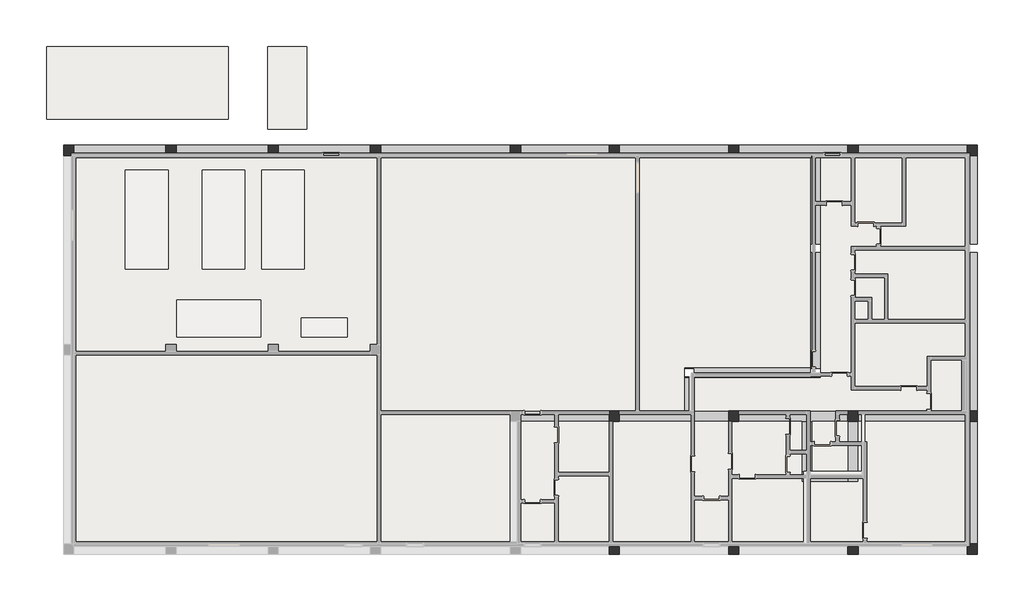
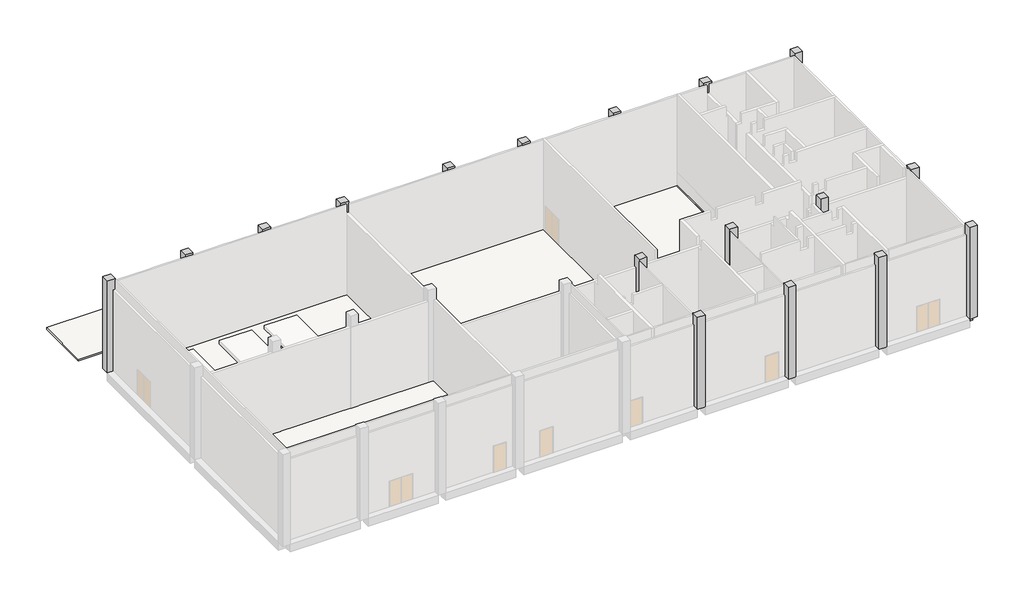
# One storey, part 4 of 4: 17 columns, 9 beams, 3 slabs.
"""IFC4 building model written with IfcOpenShell, lengths in millimetres."""

from ifc_helpers import new_model, si_unit, frame, origin, place, context, project, spatial, polyline, outline, extrude, faceted_brep, element, save

model = new_model("IFC4")

# Units and contexts
model_context = context("Model", 3, world=origin())
ifc_project = project(units=[si_unit("LENGTHUNIT", "METRE", prefix="MILLI")], contexts=[model_context])

# Site, building, storey
site = spatial("IfcSite", under=ifc_project)
building = spatial("IfcBuilding", under=site)
storey = spatial("IfcBuildingStorey", under=building, Name="TOC(GF)", Elevation=97049.9618634)

# Beams
placement = place(None, origin())
element("IfcBeam", 1, ObjectType="RC Beam_Rectangular : H_SB_AR S16_TG-UG_TG1 600x650", at=placement, inside=storey, context=model_context, shape_type="Brep", body=[
    faceted_brep([(5700.0, 3600.0, 97049.9618634), (5700.0, 4200.0, 97049.9618634), (300.0, 4200.0, 97049.9618634), (300.0, 3600.0, 97049.9618634), (5700.0, 4200.0, 96399.9618634), (300.0, 4200.0, 96399.9618634), (5700.0, 3600.0, 96399.9618634), (300.0, 3600.0, 96399.9618634), (300.0, 3600.0, 96849.9618634)], [[[0, 1, 2, 3]], [[1, 4, 5, 2]], [[4, 6, 7, 5]], [[6, 0, 3, 8, 7]], [[3, 2, 5, 7, 8]], [[1, 0, 6, 4]]]),
    faceted_brep([(6300.0, 3600.0, 97049.9618634), (6300.0, 4200.0, 97049.9618634), (6300.0, 4200.0, 96399.9618634), (6300.0, 3600.0, 96399.9618634), (11700.0, 4200.0, 97049.9618634), (11700.0, 3600.0, 97049.9618634), (11700.0, 3600.0, 96399.9618634), (11700.0, 4200.0, 96399.9618634)], [[[0, 1, 2, 3]], [[4, 5, 6, 7]], [[1, 0, 5, 4]], [[2, 1, 4, 7]], [[3, 2, 7, 6]], [[0, 3, 6, 5]]]),
    faceted_brep([(12300.0, 3600.0, 97049.9618634), (12300.0, 4200.0, 97049.9618634), (12300.0, 4200.0, 96399.9618634), (12300.0, 3600.0, 96399.9618634), (17700.0, 4200.0, 97049.9618634), (17700.0, 3600.0, 97049.9618634), (17700.0, 3600.0, 96399.9618634), (17700.0, 4200.0, 96399.9618634)], [[[0, 1, 2, 3]], [[4, 5, 6, 7]], [[1, 0, 5, 4]], [[2, 1, 4, 7]], [[3, 2, 7, 6]], [[0, 3, 6, 5]]]),
    faceted_brep([(18300.0, 3600.0, 97049.9618634), (18300.0, 4200.0, 97049.9618634), (18300.0, 4200.0, 96399.9618634), (18300.0, 3600.0, 96399.9618634), (25900.0, 3600.0, 97049.9618634), (25900.0, 4200.0, 97049.9618634), (25900.0, 4200.0, 96399.9618634), (25900.0, 3600.0, 96399.9618634)], [[[0, 1, 2, 3]], [[1, 0, 4, 5]], [[2, 1, 5, 6]], [[3, 2, 6, 7]], [[0, 3, 7, 4]], [[5, 4, 7, 6]]]),
    faceted_brep([(52700.0, 4200.0, 97049.9618634), (52700.0, 3600.0, 97049.9618634), (52700.0, 3600.0, 96849.9618634), (52700.0, 3600.0, 96399.9618634), (52700.0, 4200.0, 96399.9618634), (46300.0, 3600.0, 97049.9618634), (46300.0, 4200.0, 97049.9618634), (46300.0, 4200.0, 96399.9618634), (46300.0, 3600.0, 96399.9618634)], [[[0, 1, 2, 3, 4]], [[5, 6, 7, 8]], [[1, 0, 6, 5]], [[0, 4, 7, 6]], [[4, 3, 8, 7]], [[3, 2, 1, 5, 8]]]),
    faceted_brep([(45700.0, 4200.0, 97049.9618634), (45700.0, 3600.0, 97049.9618634), (45700.0, 3600.0, 96399.9618634), (45700.0, 4200.0, 96399.9618634), (39300.0, 3600.0, 97049.9618634), (39300.0, 4200.0, 97049.9618634), (39300.0, 4200.0, 96399.9618634), (39300.0, 3600.0, 96399.9618634), (43500.0, 3600.0, 97049.9618634), (44100.0, 3600.0, 97049.9618634), (44100.0, 3600.0, 96399.9618634), (43500.0, 3600.0, 96399.9618634)], [[[0, 1, 2, 3]], [[4, 5, 6, 7]], [[1, 0, 5, 4, 8, 9]], [[0, 3, 6, 5]], [[3, 2, 10, 11, 7, 6]], [[2, 1, 9, 8, 4, 7, 11, 10]]]),
    faceted_brep([(38700.0, 4200.0, 97049.9618634), (38700.0, 3600.0, 97049.9618634), (38700.0, 3600.0, 96399.9618634), (38700.0, 4200.0, 96399.9618634), (32300.0, 3600.0, 97049.9618634), (32300.0, 4200.0, 97049.9618634), (32300.0, 4200.0, 96399.9618634), (32300.0, 3600.0, 96399.9618634)], [[[0, 1, 2, 3]], [[4, 5, 6, 7]], [[1, 0, 5, 4]], [[0, 3, 6, 5]], [[3, 2, 7, 6]], [[2, 1, 4, 7]]]),
    faceted_brep([(31700.0, 4200.0, 97049.9618634), (31700.0, 3600.0, 97049.9618634), (31700.0, 3600.0, 96399.9618634), (31700.0, 4200.0, 96399.9618634), (26500.0, 3600.0, 97049.9618634), (26500.0, 4200.0, 97049.9618634), (26500.0, 4200.0, 96399.9618634), (26500.0, 3600.0, 96399.9618634)], [[[0, 1, 2, 3]], [[4, 5, 6, 7]], [[1, 0, 5, 4]], [[0, 3, 6, 5]], [[3, 2, 7, 6]], [[2, 1, 4, 7]]]),
])
element("IfcBeam", 2, ObjectType="RC Beam_Rectangular : H_SB_AR S16_TG-UG_TG1 600x650", at=placement, inside=storey, context=model_context, shape_type="Brep", body=[
    faceted_brep([(53300.0, 3600.0, 97049.9618634), (52700.0, 3600.0, 97049.9618634), (52700.0, -1600.0, 97049.9618634), (53300.0, -1600.0, 97049.9618634), (53300.0, -1600.0, 96399.9618634), (53300.0, 3600.0, 96399.9618634), (52700.0, 3600.0, 96399.9618634), (52700.0, -1600.0, 96399.9618634), (52700.0, 3600.0, 96849.9618634)], [[[0, 1, 2, 3]], [[3, 4, 5, 0]], [[6, 5, 4, 7]], [[1, 8, 6, 7, 2]], [[0, 5, 6, 8, 1]], [[3, 2, 7, 4]]]),
    faceted_brep([(52700.0, -19200.0, 97049.9618634), (52700.0, -19200.0, 96849.9618634), (52700.0, -19200.0, 96399.9618634), (53300.0, -19200.0, 96399.9618634), (53300.0, -19200.0, 97049.9618634), (52700.0, -12000.0, 97049.9618634), (53300.0, -12000.0, 97049.9618634), (53300.0, -12000.0, 96399.9618634), (52700.0, -12000.0, 96399.9618634), (52700.0, -12000.0, 96849.9618634)], [[[0, 1, 2, 3, 4]], [[5, 6, 7, 8, 9]], [[0, 4, 6, 5]], [[4, 3, 7, 6]], [[3, 2, 8, 7]], [[2, 1, 0, 5, 9, 8]]]),
    faceted_brep([(52700.0, -2100.0, 97049.9618634), (53300.0, -2100.0, 97049.9618634), (53300.0, -2100.0, 96399.9618634), (52700.0, -2100.0, 96399.9618634), (52700.0, -11400.0, 97049.9618634), (53300.0, -11400.0, 97049.9618634), (53300.0, -11400.0, 96399.9618634), (52700.0, -11400.0, 96399.9618634), (52700.0, -11400.0, 96849.9618634)], [[[0, 1, 2, 3]], [[1, 0, 4, 5]], [[2, 1, 5, 6]], [[3, 2, 6, 7]], [[0, 3, 7, 8, 4]], [[5, 4, 8, 7, 6]]]),
])
element("IfcBeam", 3, ObjectType="RC Beam_Rectangular : H_SB_AR S16_TG-UG_TG1 600x650", at=placement, inside=storey, context=model_context, shape_type="Brep", body=[
    faceted_brep([(43500.0, -9450.0, 97049.9618634), (44100.0, -9450.0, 97049.9618634), (44100.0, -9400.0, 97049.9618634), (43500.0, -9400.0, 97049.9618634), (43500.0, -9450.0, 96399.9618634), (43500.0, -9400.0, 96399.9618634), (44100.0, -9450.0, 96399.9618634), (44100.0, -9400.0, 96399.9618634), (44100.0, -9450.0, 96849.9618634)], [[[0, 1, 2, 3]], [[4, 0, 3, 5]], [[6, 4, 5, 7]], [[1, 8, 6, 7, 2]], [[1, 0, 4, 6, 8]], [[3, 2, 7, 5]]]),
    faceted_brep([(43500.0, 3600.0, 97049.9618634), (44100.0, 3600.0, 97049.9618634), (44100.0, 3600.0, 96849.9618634), (44100.0, 3600.0, 96399.9618634), (43500.0, 3600.0, 96399.9618634), (43500.0, 3600.0, 96849.9618634), (44100.0, -1600.0, 97049.9618634), (43500.0, -1600.0, 97049.9618634), (43500.0, -1600.0, 96399.9618634), (44100.0, -1600.0, 96399.9618634)], [[[0, 1, 2, 3, 4, 5]], [[6, 7, 8, 9]], [[1, 0, 7, 6]], [[0, 5, 4, 8, 7]], [[4, 3, 9, 8]], [[3, 2, 1, 6, 9]]]),
    faceted_brep([(43500.0, -2100.0, 97049.9618634), (44100.0, -2100.0, 97049.9618634), (44100.0, -2100.0, 96399.9618634), (43500.0, -2100.0, 96399.9618634), (44100.0, -8900.0, 97049.9618634), (43500.0, -8900.0, 97049.9618634), (43500.0, -8900.0, 96399.9618634), (44100.0, -8900.0, 96399.9618634), (43500.0, -8850.0, 97049.9618634), (43500.0, -8850.0, 96399.9618634)], [[[0, 1, 2, 3]], [[4, 5, 6, 7]], [[1, 0, 8, 5, 4]], [[0, 3, 9, 6, 5, 8]], [[3, 2, 7, 6, 9]], [[2, 1, 4, 7]]]),
])
element("IfcBeam", 4, ObjectType="RC Beam_Rectangular : H_SB_AR S16_TG-UG_TG1 600x650", at=placement, inside=storey, context=model_context, shape_type="Brep", body=[
    faceted_brep([(43500.0, -9450.0, 97049.9618634), (43500.0, -9400.0, 97049.9618634), (43500.0, -8900.0, 97049.9618634), (43500.0, -8850.0, 97049.9618634), (36100.0, -8850.0, 97049.9618634), (36100.0, -8900.0, 97049.9618634), (36700.0, -8900.0, 97049.9618634), (36700.0, -9400.0, 97049.9618634), (36100.0, -9400.0, 97049.9618634), (36100.0, -9450.0, 97049.9618634), (36700.0, -9450.0, 97049.9618634), (43500.0, -8850.0, 96849.9618634), (43500.0, -8850.0, 96399.9618634), (36100.0, -8850.0, 96399.9618634), (36100.0, -8850.0, 96849.9618634), (43500.0, -8900.0, 96399.9618634), (43500.0, -9400.0, 96399.9618634), (43500.0, -9450.0, 96399.9618634), (36700.0, -9450.0, 96399.9618634), (36100.0, -9450.0, 96399.9618634), (36100.0, -9400.0, 96399.9618634), (36700.0, -9400.0, 96399.9618634), (36700.0, -8900.0, 96399.9618634), (36100.0, -8900.0, 96399.9618634)], [[[0, 1, 2, 3, 4, 5, 6, 7, 8, 9, 10]], [[3, 11, 12, 13, 14, 4]], [[12, 15, 16, 17, 18, 19, 20, 21, 22, 23, 13]], [[9, 19, 18, 17, 0, 10]], [[3, 2, 1, 0, 17, 16, 15, 12, 11]], [[7, 21, 20, 8]], [[22, 6, 5, 23]], [[6, 22, 21, 7]], [[4, 14, 13, 23, 5]], [[19, 9, 8, 20]]]),
])
element("IfcBeam", 5, ObjectType="RC Beam_Rectangular : H_SB_AR S16_TG-UG_TG1 600x650", at=placement, inside=storey, context=model_context, shape_type="Brep", body=[
    faceted_brep([(26500.0, -11400.0, 97049.9618634), (26500.0, -12000.0, 97049.9618634), (31700.0, -12000.0, 97049.9618634), (31700.0, -11400.0, 97049.9618634), (26500.0, -12000.0, 96849.9618634), (26500.0, -12000.0, 96399.9618634), (31700.0, -12000.0, 96399.9618634), (26500.0, -11400.0, 96399.9618634), (31700.0, -11400.0, 96399.9618634)], [[[0, 1, 2, 3]], [[1, 4, 5, 6, 2]], [[5, 7, 8, 6]], [[7, 0, 3, 8]], [[1, 0, 7, 5, 4]], [[3, 2, 6, 8]]]),
    faceted_brep([(32300.0, -12000.0, 97049.9618634), (32300.0, -11400.0, 97049.9618634), (32300.0, -11400.0, 96399.9618634), (32300.0, -12000.0, 96399.9618634), (38700.0, -11400.0, 97049.9618634), (38700.0, -12000.0, 97049.9618634), (38700.0, -12000.0, 96399.9618634), (38700.0, -11400.0, 96399.9618634), (36700.0, -11400.0, 97049.9618634), (36100.0, -11400.0, 97049.9618634), (36100.0, -11400.0, 96399.9618634), (36700.0, -11400.0, 96399.9618634)], [[[0, 1, 2, 3]], [[4, 5, 6, 7]], [[1, 0, 5, 4, 8, 9]], [[0, 3, 6, 5]], [[3, 2, 10, 11, 7, 6]], [[2, 1, 9, 8, 4, 7, 11, 10]]]),
    faceted_brep([(39300.0, -12000.0, 97049.9618634), (39300.0, -11400.0, 97049.9618634), (39300.0, -11400.0, 96399.9618634), (39300.0, -12000.0, 96399.9618634), (45700.0, -11400.0, 97049.9618634), (45700.0, -12000.0, 97049.9618634), (45700.0, -12000.0, 96849.9618634), (45700.0, -12000.0, 96399.9618634), (45700.0, -11400.0, 96399.9618634), (43000.0, -12000.0, 97049.9618634), (43600.0, -12000.0, 97049.9618634), (43000.0, -12000.0, 96399.9618634), (43600.0, -12000.0, 96399.9618634)], [[[0, 1, 2, 3]], [[4, 5, 6, 7, 8]], [[4, 1, 0, 9, 10, 5]], [[5, 10, 9, 0, 3, 11, 12, 7, 6]], [[7, 12, 11, 3, 2, 8]], [[1, 4, 8, 2]]]),
    faceted_brep([(46300.0, -12000.0, 97049.9618634), (46300.0, -11400.0, 97049.9618634), (46300.0, -11400.0, 96399.9618634), (46300.0, -12000.0, 96399.9618634), (46300.0, -12000.0, 96849.9618634), (52700.0, -11400.0, 97049.9618634), (52700.0, -12000.0, 97049.9618634), (52700.0, -12000.0, 96849.9618634), (52700.0, -12000.0, 96399.9618634), (52700.0, -11400.0, 96399.9618634), (52700.0, -11400.0, 96849.9618634)], [[[0, 1, 2, 3, 4]], [[5, 6, 7, 8, 9, 10]], [[1, 0, 6, 5]], [[0, 4, 3, 8, 7, 6]], [[3, 2, 9, 8]], [[2, 1, 5, 10, 9]]]),
])
element("IfcBeam", 6, ObjectType="RC Beam_Rectangular : H_SB_AR S16_TG-UG_TG1 600x650", at=placement, inside=storey, context=model_context, shape_type="Brep", body=[
    faceted_brep([(36700.0, -9450.0, 97049.9618634), (36100.0, -9450.0, 97049.9618634), (36100.0, -11400.0, 97049.9618634), (36700.0, -11400.0, 97049.9618634), (36100.0, -9450.0, 96399.9618634), (36100.0, -11400.0, 96399.9618634), (36100.0, -11400.0, 96849.9618634), (36700.0, -9450.0, 96399.9618634), (36700.0, -11400.0, 96399.9618634), (36700.0, -9450.0, 96849.9618634), (36700.0, -11400.0, 96849.9618634)], [[[0, 1, 2, 3]], [[1, 4, 5, 6, 2]], [[4, 7, 8, 5]], [[7, 9, 0, 3, 10, 8]], [[1, 0, 9, 7, 4]], [[3, 2, 6, 5, 8, 10]]]),
])
element("IfcBeam", 7, ObjectType="RC Beam_Rectangular : H_SB_AR S16_TG-UG_TG1 600x650", at=placement, inside=storey, context=model_context, shape_type="Brep", body=[
    faceted_brep([(45700.0, -15550.0, 97049.9618634), (46300.0, -15550.0, 97049.9618634), (46300.0, -12000.0, 97049.9618634), (45700.0, -12000.0, 97049.9618634), (45700.0, -14950.0, 97049.9618634), (45700.0, -15550.0, 96399.9618634), (45700.0, -12000.0, 96849.9618634), (45700.0, -12000.0, 96399.9618634), (45700.0, -14950.0, 96399.9618634), (46300.0, -15550.0, 96399.9618634), (46300.0, -12000.0, 96399.9618634), (46300.0, -15550.0, 96849.9618634), (46300.0, -12000.0, 96849.9618634)], [[[0, 1, 2, 3, 4]], [[5, 0, 4, 3, 6, 7, 8]], [[9, 5, 8, 7, 10]], [[1, 11, 9, 10, 12, 2]], [[1, 0, 5, 9, 11]], [[3, 2, 12, 10, 7, 6]]]),
])
element("IfcBeam", 8, ObjectType="RC Beam_Rectangular : H_SB_AR S16_TG-UG_TG1 600x650", at=placement, inside=storey, context=model_context, shape_type="Brep", body=[
    faceted_brep([(43000.0, -14950.0, 97049.9618634), (43000.0, -15550.0, 97049.9618634), (45700.0, -15550.0, 97049.9618634), (45700.0, -14950.0, 97049.9618634), (43600.0, -14950.0, 97049.9618634), (43000.0, -14950.0, 96399.9618634), (45700.0, -14950.0, 96849.9618634), (45700.0, -14950.0, 96399.9618634), (43600.0, -14950.0, 96399.9618634), (43000.0, -15550.0, 96399.9618634), (45700.0, -15550.0, 96399.9618634), (43000.0, -15550.0, 96849.9618634)], [[[0, 1, 2, 3, 4]], [[5, 0, 4, 3, 6, 7, 8]], [[9, 5, 8, 7, 10]], [[1, 11, 9, 10, 2]], [[3, 2, 10, 7, 6]], [[1, 0, 5, 9, 11]]]),
])
element("IfcBeam", 9, ObjectType="RC Beam_Rectangular : H_SB_AR S16_TG-UG_TG1 600x650", at=placement, inside=storey, context=model_context, shape_type="Brep", body=[
    faceted_brep([(43000.0, -14950.0, 97049.9618634), (43600.0, -14950.0, 97049.9618634), (43600.0, -12000.0, 97049.9618634), (43000.0, -12000.0, 97049.9618634), (43600.0, -14950.0, 96849.9618634), (43600.0, -14950.0, 96399.9618634), (43600.0, -12000.0, 96399.9618634), (43600.0, -12000.0, 96849.9618634), (43000.0, -14950.0, 96399.9618634), (43000.0, -12000.0, 96399.9618634), (43000.0, -12000.0, 96849.9618634)], [[[0, 1, 2, 3]], [[1, 4, 5, 6, 7, 2]], [[5, 8, 9, 6]], [[8, 0, 3, 10, 9]], [[1, 0, 8, 5, 4]], [[3, 2, 7, 6, 9, 10]]]),
])

# Columns
element("IfcColumn", 10, ObjectType="RC_Column_Rectangular : H_SC_AR S15_RC Col-AG_C1 600x600", at=placement, inside=storey, context=model_context, shape_type="Brep", body=[
    faceted_brep([(300.0, 4200.0, 97049.9618634), (300.0, 3600.0, 97049.9618634), (-300.0, 3600.0, 97049.9618634), (-300.0, 4200.0, 97049.9618634), (300.0, 4200.0, 104550.0), (300.0, 3600.0, 104550.0), (300.0, 3600.0, 103650.0), (300.0, 4200.0, 103650.0), (-300.0, 3600.0, 104550.0), (-300.0, 3600.0, 103650.0), (-300.0, 4200.0, 104550.0)], [[[0, 1, 2, 3]], [[4, 5, 6, 1, 0, 7]], [[5, 8, 9, 2, 1, 6]], [[8, 10, 3, 2, 9]], [[10, 4, 7, 0, 3]], [[4, 10, 8, 5]]]),
])
element("IfcColumn", 11, ObjectType="RC_Column_Rectangular : H_SC_AR S15_RC Col-AG_C1 600x600", at=placement, inside=storey, context=model_context, shape_type="Brep", body=[
    faceted_brep([(32300.0, -19200.0, 97049.9618634), (32300.0, -19800.0, 97049.9618634), (31700.0, -19800.0, 97049.9618634), (31700.0, -19200.0, 97049.9618634), (32300.0, -19200.0, 104550.0), (32300.0, -19800.0, 104550.0), (32300.0, -19800.0, 103650.0), (32300.0, -19200.0, 103650.0), (31700.0, -19800.0, 104550.0), (31700.0, -19800.0, 103650.0), (31700.0, -19200.0, 104550.0), (31700.0, -19200.0, 103650.0), (31750.0, -19200.0, 104550.0), (32250.0, -19200.0, 104550.0)], [[[0, 1, 2, 3]], [[4, 5, 6, 1, 0, 7]], [[5, 8, 9, 2, 1, 6]], [[8, 10, 11, 3, 2, 9]], [[10, 12, 13, 4, 7, 0, 3, 11]], [[4, 13, 12, 10, 8, 5]]]),
])
element("IfcColumn", 12, ObjectType="RC_Column_Rectangular : H_SC_AR S15_RC Col-AG_C1 600x600", at=placement, inside=storey, context=model_context, shape_type="Brep", body=[
    faceted_brep([(39300.0, -19200.0, 97049.9618634), (39300.0, -19800.0, 97049.9618634), (38700.0, -19800.0, 97049.9618634), (38700.0, -19200.0, 97049.9618634), (39300.0, -19200.0, 104550.0), (39300.0, -19800.0, 104550.0), (39300.0, -19800.0, 103650.0), (39300.0, -19200.0, 103650.0), (38700.0, -19800.0, 104550.0), (38700.0, -19800.0, 103650.0), (38700.0, -19200.0, 104550.0), (38700.0, -19200.0, 103650.0), (38750.0, -19200.0, 104550.0), (39250.0, -19200.0, 104550.0)], [[[0, 1, 2, 3]], [[4, 5, 6, 1, 0, 7]], [[5, 8, 9, 2, 1, 6]], [[8, 10, 11, 3, 2, 9]], [[10, 12, 13, 4, 7, 0, 3, 11]], [[4, 13, 12, 10, 8, 5]]]),
])
element("IfcColumn", 13, ObjectType="RC_Column_Rectangular : H_SC_AR S15_RC Col-AG_C1 600x600", at=placement, inside=storey, context=model_context, shape_type="Brep", body=[
    faceted_brep([(46300.0, -19200.0, 97049.9618634), (46300.0, -19800.0, 97049.9618634), (45700.0, -19800.0, 97049.9618634), (45700.0, -19200.0, 97049.9618634), (46300.0, -19200.0, 104550.0), (46300.0, -19800.0, 104550.0), (46300.0, -19800.0, 103650.0), (46300.0, -19200.0, 103650.0), (45700.0, -19800.0, 104550.0), (45700.0, -19800.0, 103650.0), (45700.0, -19200.0, 104550.0), (45700.0, -19200.0, 103650.0), (45750.0, -19200.0, 104550.0), (46250.0, -19200.0, 104550.0)], [[[0, 1, 2, 3]], [[4, 5, 6, 1, 0, 7]], [[5, 8, 9, 2, 1, 6]], [[8, 10, 11, 3, 2, 9]], [[10, 12, 13, 4, 7, 0, 3, 11]], [[4, 13, 12, 10, 8, 5]]]),
])
element("IfcColumn", 14, ObjectType="RC_Column_Rectangular : H_SC_AR S15_RC Col-AG_C1 600x600", at=placement, inside=storey, context=model_context, shape_type="Brep", body=[
    faceted_brep([(53300.0, -19200.0, 97049.9618634), (53300.0, -19800.0, 97049.9618634), (52700.0, -19800.0, 97049.9618634), (52700.0, -19200.0, 97049.9618634), (53300.0, -19200.0, 104550.0), (53300.0, -19800.0, 104550.0), (53300.0, -19200.0, 103650.0), (52700.0, -19800.0, 104550.0), (52700.0, -19800.0, 103650.0), (52700.0, -19200.0, 104550.0), (52700.0, -19200.0, 103650.0)], [[[0, 1, 2, 3]], [[4, 5, 1, 0, 6]], [[5, 7, 8, 2, 1]], [[7, 9, 10, 3, 2, 8]], [[9, 4, 6, 0, 3, 10]], [[4, 9, 7, 5]]]),
])
element("IfcColumn", 15, ObjectType="RC_Column_Rectangular : H_SC_AR S15_RC Col-AG_C1 600x600", at=placement, inside=storey, context=model_context, shape_type="Brep", body=[
    faceted_brep([(6300.0, 4200.0, 97049.9618634), (6300.0, 3600.0, 97049.9618634), (5700.0, 3600.0, 97049.9618634), (5700.0, 4200.0, 97049.9618634), (6300.0, 4200.0, 104550.0), (6300.0, 3600.0, 104550.0), (6300.0, 3600.0, 103650.0), (6300.0, 4200.0, 103650.0), (6200.0, 3600.0, 104550.0), (5800.0, 3600.0, 104550.0), (5700.0, 3600.0, 104550.0), (5700.0, 3600.0, 103650.0), (5700.0, 4200.0, 104550.0), (5700.0, 4200.0, 103650.0)], [[[0, 1, 2, 3]], [[4, 5, 6, 1, 0, 7]], [[5, 8, 9, 10, 11, 2, 1, 6]], [[10, 12, 13, 3, 2, 11]], [[12, 4, 7, 0, 3, 13]], [[4, 12, 10, 9, 8, 5]]]),
])
element("IfcColumn", 16, ObjectType="RC_Column_Rectangular : H_SC_AR S15_RC Col-AG_C1 600x600", at=placement, inside=storey, context=model_context, shape_type="Brep", body=[
    faceted_brep([(12300.0, 4200.0, 97049.9618634), (12300.0, 3600.0, 97049.9618634), (11700.0, 3600.0, 97049.9618634), (11700.0, 4200.0, 97049.9618634), (12300.0, 4200.0, 104550.0), (12300.0, 3600.0, 104550.0), (12300.0, 3600.0, 103650.0), (12300.0, 4200.0, 103650.0), (12200.0, 3600.0, 104550.0), (11800.0, 3600.0, 104550.0), (11700.0, 3600.0, 104550.0), (11700.0, 3600.0, 103650.0), (11700.0, 4200.0, 104550.0), (11700.0, 4200.0, 103650.0)], [[[0, 1, 2, 3]], [[4, 5, 6, 1, 0, 7]], [[5, 8, 9, 10, 11, 2, 1, 6]], [[10, 12, 13, 3, 2, 11]], [[12, 4, 7, 0, 3, 13]], [[4, 12, 10, 9, 8, 5]]]),
])
element("IfcColumn", 17, ObjectType="RC_Column_Rectangular : H_SC_AR S15_RC Col-AG_C1 600x600", at=placement, inside=storey, context=model_context, shape_type="Brep", body=[
    faceted_brep([(18300.0, 4200.0, 97049.9618634), (18300.0, 3600.0, 97049.9618634), (17700.0, 3600.0, 97049.9618634), (17700.0, 4200.0, 97049.9618634), (18300.0, 4200.0, 104550.0), (18300.0, 3600.0, 104550.0), (18300.0, 3600.0, 103650.0), (18300.0, 4200.0, 103650.0), (17700.0, 3600.0, 104550.0), (17700.0, 3600.0, 103650.0), (17700.0, 4200.0, 104550.0), (17700.0, 4200.0, 103650.0)], [[[0, 1, 2, 3]], [[4, 5, 6, 1, 0, 7]], [[5, 8, 9, 2, 1, 6]], [[8, 10, 11, 3, 2, 9]], [[10, 4, 7, 0, 3, 11]], [[4, 10, 8, 5]]]),
])
element("IfcColumn", 18, ObjectType="RC_Column_Rectangular : H_SC_AR S15_RC Col-AG_C2 600x600 2", at=placement, inside=storey, context=model_context, shape_type="Brep", body=[
    faceted_brep([(32300.0, -11400.0, 97049.9618634), (32300.0, -12000.0, 97049.9618634), (31700.0, -12000.0, 97049.9618634), (31700.0, -11400.0, 97049.9618634), (32300.0, -11400.0, 104550.0), (32300.0, -12000.0, 104550.0), (32300.0, -12000.0, 103650.0), (32300.0, -11400.0, 103650.0), (32250.0, -12000.0, 104550.0), (31750.0, -12000.0, 104550.0), (31700.0, -12000.0, 104550.0), (31700.0, -12000.0, 103650.0), (31700.0, -11400.0, 104550.0), (31700.0, -11400.0, 103650.0), (31750.0, -11400.0, 104550.0), (32250.0, -11400.0, 104550.0)], [[[0, 1, 2, 3]], [[4, 5, 6, 1, 0, 7]], [[5, 8, 9, 10, 11, 2, 1, 6]], [[10, 12, 13, 3, 2, 11]], [[12, 14, 15, 4, 7, 0, 3, 13]], [[4, 15, 14, 12, 10, 9, 8, 5]]]),
])
element("IfcColumn", 19, ObjectType="RC_Column_Rectangular : H_SC_AR S15_RC Col-AG_C2 600x600 2", at=placement, inside=storey, context=model_context, shape_type="Brep", body=[
    faceted_brep([(39300.0, -11400.0, 97049.9618634), (39300.0, -12000.0, 97049.9618634), (38700.0, -12000.0, 97049.9618634), (38700.0, -11400.0, 97049.9618634), (39300.0, -11400.0, 104550.0), (39300.0, -12000.0, 104550.0), (39300.0, -12000.0, 103650.0), (39300.0, -11400.0, 103650.0), (39250.0, -12000.0, 104550.0), (38750.0, -12000.0, 104550.0), (38700.0, -12000.0, 104550.0), (38700.0, -12000.0, 103650.0), (38700.0, -11400.0, 104550.0), (38700.0, -11400.0, 103650.0), (38750.0, -11400.0, 104550.0), (39250.0, -11400.0, 104550.0)], [[[0, 1, 2, 3]], [[4, 5, 6, 1, 0, 7]], [[5, 8, 9, 10, 11, 2, 1, 6]], [[10, 12, 13, 3, 2, 11]], [[12, 14, 15, 4, 7, 0, 3, 13]], [[4, 15, 14, 12, 10, 9, 8, 5]]]),
])
element("IfcColumn", 20, ObjectType="RC_Column_Rectangular : H_SC_AR S15_RC Col-AG_C2 600x600 2", at=placement, inside=storey, context=model_context, shape_type="Brep", body=[
    faceted_brep([(46300.0, -11400.0, 97049.9618634), (46300.0, -12000.0, 97049.9618634), (45700.0, -12000.0, 97049.9618634), (45700.0, -11400.0, 97049.9618634), (46300.0, -11400.0, 104550.0), (46300.0, -12000.0, 104550.0), (46300.0, -12000.0, 103650.0), (46300.0, -11400.0, 103650.0), (46250.0, -12000.0, 104550.0), (45750.0, -12000.0, 104550.0), (45700.0, -12000.0, 104550.0), (45700.0, -12000.0, 103650.0), (45700.0, -11400.0, 104550.0), (45700.0, -11400.0, 103650.0), (45750.0, -11400.0, 104550.0), (46250.0, -11400.0, 104550.0)], [[[0, 1, 2, 3]], [[4, 5, 6, 1, 0, 7]], [[5, 8, 9, 10, 11, 2, 1, 6]], [[10, 12, 13, 3, 2, 11]], [[12, 14, 15, 4, 7, 0, 3, 13]], [[4, 15, 14, 12, 10, 9, 8, 5]]]),
])
element("IfcColumn", 21, ObjectType="RC_Column_Rectangular : H_SC_AR S15_RC Col-AG_C2 600x600 2", at=placement, inside=storey, context=model_context, shape_type="Brep", body=[
    faceted_brep([(53300.0, -11400.0, 97049.9618634), (53300.0, -12000.0, 97049.9618634), (52700.0, -12000.0, 97049.9618634), (52700.0, -11400.0, 97049.9618634), (53300.0, -11400.0, 104550.0), (53300.0, -12000.0, 104550.0), (53300.0, -12000.0, 103650.0), (53300.0, -11400.0, 103650.0), (52700.0, -12000.0, 104550.0), (52700.0, -12000.0, 103650.0), (52700.0, -11400.0, 104550.0), (52700.0, -11400.0, 103650.0)], [[[0, 1, 2, 3]], [[4, 5, 6, 1, 0, 7]], [[5, 8, 9, 2, 1, 6]], [[8, 10, 11, 3, 2, 9]], [[10, 4, 7, 0, 3, 11]], [[4, 10, 8, 5]]]),
])
element("IfcColumn", 22, ObjectType="RC_Column_Rectangular : H_SC_AR S15_RC Col-AG_C2 600x600 2", at=placement, inside=storey, context=model_context, shape_type="Brep", body=[
    faceted_brep([(53300.0, 4200.0, 97049.9618634), (53300.0, 3600.0, 97049.9618634), (52700.0, 3600.0, 97049.9618634), (52700.0, 4200.0, 97049.9618634), (53300.0, 4200.0, 104550.0), (53300.0, 3600.0, 104550.0), (53300.0, 3600.0, 103650.0), (52700.0, 3600.0, 104550.0), (52700.0, 3600.0, 103650.0), (52700.0, 4200.0, 104550.0), (52700.0, 4200.0, 103650.0)], [[[0, 1, 2, 3]], [[4, 5, 6, 1, 0]], [[5, 7, 8, 2, 1, 6]], [[7, 9, 10, 3, 2, 8]], [[9, 4, 0, 3, 10]], [[4, 9, 7, 5]]]),
])
element("IfcColumn", 23, ObjectType="RC_Column_Rectangular : H_SC_AR S15_RC Col-AG_C2 600x600 2", at=placement, inside=storey, context=model_context, shape_type="Brep", body=[
    faceted_brep([(46300.0, 4200.0, 97049.9618634), (46300.0, 3600.0, 97049.9618634), (45700.0, 3600.0, 97049.9618634), (45700.0, 4200.0, 97049.9618634), (46300.0, 4200.0, 104550.0), (46300.0, 3600.0, 104550.0), (46300.0, 3600.0, 103650.0), (46300.0, 4200.0, 103650.0), (46250.0, 3600.0, 104550.0), (45750.0, 3600.0, 104550.0), (45700.0, 3600.0, 104550.0), (45700.0, 3600.0, 103650.0), (45700.0, 4200.0, 104550.0), (45700.0, 4200.0, 103650.0)], [[[0, 1, 2, 3]], [[4, 5, 6, 1, 0, 7]], [[5, 8, 9, 10, 11, 2, 1, 6]], [[10, 12, 13, 3, 2, 11]], [[12, 4, 7, 0, 3, 13]], [[4, 12, 10, 9, 8, 5]]]),
])
element("IfcColumn", 24, ObjectType="RC_Column_Rectangular : H_SC_AR S15_RC Col-AG_C2 600x600 2", at=placement, inside=storey, context=model_context, shape_type="Brep", body=[
    faceted_brep([(39300.0, 4200.0, 97049.9618634), (39300.0, 3600.0, 97049.9618634), (38700.0, 3600.0, 97049.9618634), (38700.0, 4200.0, 97049.9618634), (39300.0, 4200.0, 104550.0), (39300.0, 3600.0, 104550.0), (39300.0, 3600.0, 103650.0), (39300.0, 4200.0, 103650.0), (39250.0, 3600.0, 104550.0), (38750.0, 3600.0, 104550.0), (38700.0, 3600.0, 104550.0), (38700.0, 3600.0, 103650.0), (38700.0, 4200.0, 104550.0), (38700.0, 4200.0, 103650.0)], [[[0, 1, 2, 3]], [[4, 5, 6, 1, 0, 7]], [[5, 8, 9, 10, 11, 2, 1, 6]], [[10, 12, 13, 3, 2, 11]], [[12, 4, 7, 0, 3, 13]], [[4, 12, 10, 9, 8, 5]]]),
])
element("IfcColumn", 25, ObjectType="RC_Column_Rectangular : H_SC_AR S15_RC Col-AG_C2 600x600 2", at=placement, inside=storey, context=model_context, shape_type="Brep", body=[
    faceted_brep([(32300.0, 4200.0, 97049.9618634), (32300.0, 3600.0, 97049.9618634), (31700.0, 3600.0, 97049.9618634), (31700.0, 4200.0, 97049.9618634), (32300.0, 4200.0, 104550.0), (32300.0, 3600.0, 104550.0), (32300.0, 3600.0, 103650.0), (32300.0, 4200.0, 103650.0), (32250.0, 3600.0, 104550.0), (31750.0, 3600.0, 104550.0), (31700.0, 3600.0, 104550.0), (31700.0, 3600.0, 103650.0), (31700.0, 4200.0, 104550.0), (31700.0, 4200.0, 103650.0)], [[[0, 1, 2, 3]], [[4, 5, 6, 1, 0, 7]], [[5, 8, 9, 10, 11, 2, 1, 6]], [[10, 12, 13, 3, 2, 11]], [[12, 4, 7, 0, 3, 13]], [[4, 12, 10, 9, 8, 5]]]),
])
element("IfcColumn", 26, ObjectType="RC_Column_Rectangular : H_SC_AR S15_RC Col-AG_C2 600x600 2", at=placement, inside=storey, context=model_context, shape_type="Brep", body=[
    faceted_brep([(26500.0, 4200.0, 97049.9618634), (26500.0, 3600.0, 97049.9618634), (25900.0, 3600.0, 97049.9618634), (25900.0, 4200.0, 97049.9618634), (26500.0, 4200.0, 104550.0), (26500.0, 3600.0, 104550.0), (26500.0, 3600.0, 103650.0), (26500.0, 4200.0, 103650.0), (26450.0, 3600.0, 104550.0), (25950.0, 3600.0, 104550.0), (25900.0, 3600.0, 104550.0), (25900.0, 3600.0, 103650.0), (25900.0, 4200.0, 104550.0), (25900.0, 4200.0, 103650.0)], [[[0, 1, 2, 3]], [[4, 5, 6, 1, 0, 7]], [[5, 8, 9, 10, 11, 2, 1, 6]], [[10, 12, 13, 3, 2, 11]], [[12, 4, 7, 0, 3, 13]], [[4, 12, 10, 9, 8, 5]]]),
])

# Slabs
element("IfcSlab", 27, ObjectType="H_SF_AR S17_SOG_T150 GS1", at=placement, inside=storey, context=model_context, shape_type="Brep", body=[
    faceted_brep([(300.0, -19200.0, 96849.9618634), (300.0, 3600.0, 96849.9618634), (43500.0, 3600.0, 96849.9618634), (43500.0, -1600.0, 96849.9618634), (43500.0, -2100.0, 96849.9618634), (43500.0, -8850.0, 96849.9618634), (36700.0, -8850.0, 96849.9618634), (36100.0, -8850.0, 96849.9618634), (36100.0, -8900.0, 96849.9618634), (36100.0, -9400.0, 96849.9618634), (36100.0, -11400.0, 96849.9618634), (32300.0, -11400.0, 96849.9618634), (31700.0, -11400.0, 96849.9618634), (25900.0, -11400.0, 96849.9618634), (25900.0, -19200.0, 96849.9618634), (6300.0, -8100.0, 96849.9618634), (6300.0, -7500.0, 96849.9618634), (5700.0, -7500.0, 96849.9618634), (5700.0, -8100.0, 96849.9618634), (12300.0, -8100.0, 96849.9618634), (12300.0, -7500.0, 96849.9618634), (11700.0, -7500.0, 96849.9618634), (11700.0, -8100.0, 96849.9618634), (18300.0, -8100.0, 96849.9618634), (18300.0, -7500.0, 96849.9618634), (17700.0, -7500.0, 96849.9618634), (17700.0, -8100.0, 96849.9618634), (300.0, 3600.0, 97049.9618634), (300.0, -7500.0, 97049.9618634), (300.0, -8100.0, 97049.9618634), (300.0, -19200.0, 97049.9618634), (5700.0, -19200.0, 97049.9618634), (6300.0, -19200.0, 97049.9618634), (11700.0, -19200.0, 97049.9618634), (12300.0, -19200.0, 97049.9618634), (17700.0, -19200.0, 97049.9618634), (18300.0, -19200.0, 97049.9618634), (25900.0, -19200.0, 97049.9618634), (25900.0, -12000.0, 97049.9618634), (25900.0, -11400.0, 97049.9618634), (26500.0, -11400.0, 97049.9618634), (31700.0, -11400.0, 97049.9618634), (32300.0, -11400.0, 97049.9618634), (36100.0, -11400.0, 97049.9618634), (36100.0, -9450.0, 97049.9618634), (36100.0, -9400.0, 97049.9618634), (36100.0, -8900.0, 97049.9618634), (36100.0, -8850.0, 97049.9618634), (36700.0, -8850.0, 97049.9618634), (43500.0, -8850.0, 97049.9618634), (43500.0, -2100.0, 97049.9618634), (43500.0, -1600.0, 97049.9618634), (43500.0, 3600.0, 97049.9618634), (39300.0, 3600.0, 97049.9618634), (38700.0, 3600.0, 97049.9618634), (32300.0, 3600.0, 97049.9618634), (31700.0, 3600.0, 97049.9618634), (26500.0, 3600.0, 97049.9618634), (25900.0, 3600.0, 97049.9618634), (18300.0, 3600.0, 97049.9618634), (17700.0, 3600.0, 97049.9618634), (12300.0, 3600.0, 97049.9618634), (11700.0, 3600.0, 97049.9618634), (6300.0, 3600.0, 97049.9618634), (5700.0, 3600.0, 97049.9618634), (6300.0, -7500.0, 97049.9618634), (6300.0, -8100.0, 97049.9618634), (5700.0, -8100.0, 97049.9618634), (5700.0, -7500.0, 97049.9618634), (12300.0, -7500.0, 97049.9618634), (12300.0, -8100.0, 97049.9618634), (11700.0, -8100.0, 97049.9618634), (11700.0, -7500.0, 97049.9618634), (18300.0, -7500.0, 97049.9618634), (18300.0, -8100.0, 97049.9618634), (17700.0, -8100.0, 97049.9618634), (17700.0, -7500.0, 97049.9618634)], [[[0, 1, 2, 3, 4, 5, 6, 7, 8, 9, 10, 11, 12, 13, 14], [15, 16, 17, 18], [19, 20, 21, 22], [23, 24, 25, 26]], [[27, 28, 29, 30, 31, 32, 33, 34, 35, 36, 37, 38, 39, 40, 41, 42, 43, 44, 45, 46, 47, 48, 49, 50, 51, 52, 53, 54, 55, 56, 57, 58, 59, 60, 61, 62, 63, 64], [65, 66, 67, 68], [69, 70, 71, 72], [73, 74, 75, 76]], [[1, 27, 64, 63, 62, 61, 60, 59, 58, 57, 56, 55, 54, 53, 52, 2]], [[30, 0, 14, 37, 36, 35, 34, 33, 32, 31]], [[1, 0, 30, 29, 28, 27]], [[2, 52, 51, 50, 49, 5, 4, 3]], [[5, 49, 48, 47, 7, 6]], [[10, 43, 42, 41, 40, 39, 13, 12, 11]], [[37, 14, 13, 39, 38]], [[15, 66, 65, 16]], [[66, 15, 18, 67]], [[67, 18, 17, 68]], [[68, 17, 16, 65]], [[19, 70, 69, 20]], [[70, 19, 22, 71]], [[71, 22, 21, 72]], [[72, 21, 20, 69]], [[23, 74, 73, 24]], [[74, 23, 26, 75]], [[75, 26, 25, 76]], [[76, 25, 24, 73]], [[43, 10, 9, 8, 7, 47, 46, 45, 44]]]),
    faceted_brep([(36100.0, -12000.0, 96849.9618634), (36700.0, -12000.0, 96849.9618634), (38700.0, -12000.0, 96849.9618634), (39300.0, -12000.0, 96849.9618634), (43000.0, -12000.0, 96849.9618634), (43000.0, -15550.0, 96849.9618634), (43600.0, -15550.0, 96849.9618634), (46300.0, -15550.0, 96849.9618634), (46300.0, -14950.0, 96849.9618634), (46300.0, -12000.0, 96849.9618634), (52700.0, -12000.0, 96849.9618634), (52700.0, -19200.0, 96849.9618634), (26500.0, -19200.0, 96849.9618634), (26500.0, -12000.0, 96849.9618634), (31700.0, -12000.0, 96849.9618634), (32300.0, -12000.0, 96849.9618634), (36700.0, -12000.0, 97049.9618634), (36100.0, -12000.0, 97049.9618634), (32300.0, -12000.0, 97049.9618634), (31700.0, -12000.0, 97049.9618634), (26500.0, -12000.0, 97049.9618634), (26500.0, -19200.0, 97049.9618634), (31700.0, -19200.0, 97049.9618634), (32300.0, -19200.0, 97049.9618634), (38700.0, -19200.0, 97049.9618634), (39300.0, -19200.0, 97049.9618634), (45700.0, -19200.0, 97049.9618634), (46300.0, -19200.0, 97049.9618634), (52700.0, -19200.0, 97049.9618634), (52700.0, -12000.0, 97049.9618634), (46300.0, -12000.0, 97049.9618634), (46300.0, -14950.0, 97049.9618634), (46300.0, -15550.0, 97049.9618634), (45700.0, -15550.0, 97049.9618634), (43600.0, -15550.0, 97049.9618634), (43000.0, -15550.0, 97049.9618634), (43000.0, -14950.0, 97049.9618634), (43000.0, -12000.0, 97049.9618634), (39300.0, -12000.0, 97049.9618634), (38700.0, -12000.0, 97049.9618634)], [[[0, 1, 2, 3, 4, 5, 6, 7, 8, 9, 10, 11, 12, 13, 14, 15]], [[16, 17, 18, 19, 20, 21, 22, 23, 24, 25, 26, 27, 28, 29, 30, 31, 32, 33, 34, 35, 36, 37, 38, 39]], [[21, 12, 11, 28, 27, 26, 25, 24, 23, 22]], [[1, 0, 15, 14, 13, 20, 19, 18, 17, 16, 39, 38, 37, 4, 3, 2]], [[29, 10, 9, 30]], [[13, 12, 21, 20]], [[11, 10, 29, 28]], [[7, 32, 31, 30, 9, 8]], [[32, 7, 6, 5, 35, 34, 33]], [[35, 5, 4, 37, 36]]]),
    faceted_brep([(36700.0, -11400.0, 96849.9618634), (36700.0, -9450.0, 96849.9618634), (44100.0, -9450.0, 96849.9618634), (44100.0, -9400.0, 96849.9618634), (44100.0, -8900.0, 96849.9618634), (44100.0, -8850.0, 96849.9618634), (44100.0, -2100.0, 96849.9618634), (44100.0, -1600.0, 96849.9618634), (44100.0, 3600.0, 96849.9618634), (52700.0, 3600.0, 96849.9618634), (52700.0, -11400.0, 96849.9618634), (46300.0, -11400.0, 96849.9618634), (45700.0, -11400.0, 96849.9618634), (43600.0, -11400.0, 96849.9618634), (43000.0, -11400.0, 96849.9618634), (39300.0, -11400.0, 96849.9618634), (38700.0, -11400.0, 96849.9618634), (36700.0, -9450.0, 97049.9618634), (36700.0, -11400.0, 97049.9618634), (38700.0, -11400.0, 97049.9618634), (39300.0, -11400.0, 97049.9618634), (43000.0, -11400.0, 97049.9618634), (43600.0, -11400.0, 97049.9618634), (45700.0, -11400.0, 97049.9618634), (46300.0, -11400.0, 97049.9618634), (52700.0, -11400.0, 97049.9618634), (52700.0, -2100.0, 97049.9618634), (52700.0, -1600.0, 97049.9618634), (52700.0, 3600.0, 97049.9618634), (46300.0, 3600.0, 97049.9618634), (45700.0, 3600.0, 97049.9618634), (44100.0, 3600.0, 97049.9618634), (44100.0, -1600.0, 97049.9618634), (44100.0, -2100.0, 97049.9618634), (44100.0, -8850.0, 97049.9618634), (44100.0, -8900.0, 97049.9618634), (44100.0, -9400.0, 97049.9618634), (44100.0, -9450.0, 97049.9618634), (43500.0, -9450.0, 97049.9618634)], [[[0, 1, 2, 3, 4, 5, 6, 7, 8, 9, 10, 11, 12, 13, 14, 15, 16]], [[17, 18, 19, 20, 21, 22, 23, 24, 25, 26, 27, 28, 29, 30, 31, 32, 33, 34, 35, 36, 37, 38]], [[8, 31, 30, 29, 28, 9]], [[18, 0, 16, 15, 14, 13, 12, 11, 10, 25, 24, 23, 22, 21, 20, 19]], [[1, 0, 18, 17]], [[31, 8, 7, 6, 5, 4, 3, 2, 37, 36, 35, 34, 33, 32]], [[10, 9, 28, 27, 26, 25]], [[37, 2, 1, 17, 38]]]),
    faceted_brep([(45700.0, -12000.0, 96849.9618634), (45700.0, -14950.0, 96849.9618634), (43600.0, -14950.0, 96849.9618634), (43600.0, -12000.0, 96849.9618634), (45700.0, -14950.0, 97049.9618634), (45700.0, -12000.0, 97049.9618634), (43600.0, -12000.0, 97049.9618634), (43600.0, -14950.0, 97049.9618634)], [[[0, 1, 2, 3]], [[4, 5, 6, 7]], [[5, 0, 3, 6]], [[0, 5, 4, 1]], [[1, 4, 7, 2]], [[3, 2, 7, 6]]]),
])
element("IfcSlab", 28, ObjectType="H_SF_AR B01_EQ Fdn_EF1 10650x4250x150", at=placement, inside=storey, context=model_context, shape_type="SweptSolid", body=[
    extrude(outline(polyline([(9350.0, 10000.0), (9350.0, 5750.0), (-1300.0, 5750.0), (-1300.0, 10000.0), (9350.0, 10000.0)])), frame((0.0, 0.0, 97049.9618634), z_axis=(0.0, 0.0, 1.0), x_axis=(1.0, 0.0, 0.0)), (0.0, 0.0, 1.0), 150.0),
])
element("IfcSlab", 29, ObjectType="H_SF_AR B01_EQ Fdn_EF2 2300x4850x150", at=placement, inside=storey, context=model_context, shape_type="SweptSolid", body=[
    extrude(outline(polyline([(13975.0, 5150.0), (11675.0, 5150.0), (11675.0, 10000.0), (13975.0, 10000.0), (13975.0, 5150.0)])), frame((0.0, 0.0, 97049.9618634), z_axis=(0.0, 0.0, 1.0), x_axis=(1.0, 0.0, 0.0)), (0.0, 0.0, 1.0), 150.0),
])

save(model, "model.ifc")

# Revit data of these elements
# Type "RC Beam_Rectangular : H_SB_AR S16_TG-UG_TG1 600x650"
#   Type Comments = "UG"
#   Type Mark = "TG1"
#   중앙부 하부근 = ""
#   중앙부 상부근 = ""
#   중앙부 보조근 = ""
#   중앙부 늑근 = ""
#   외단부 하부근 = ""
#   외단부 상부근 = ""
#   외단부 보조근 = ""
#   외단부 늑근 = ""
#   부호 = ""
#   내단부 하부근 = ""
#   내단부 상부근 = ""
#   내단부 보조근 = ""
#   내단부 늑근 = ""
#   ALL 하부근 = ""
#   ALL 상부근 = ""
#   ALL 보조근 = ""
#   ALL 늑근 = ""
#   H_Rebar Ratio = 0.15
#   Width = 600 mm
#   Height = 650 mm
#   Length [instance default] = 1524 mm
#   b = 600 mm
#   h = 650 mm
#   hec_material3 [instance default] = none
#   hec_material2 [instance default] = none
#   hec_material1 [instance default] = none
#   Structural Material [instance default] = none
#   Assembly Code = ""
# Type "RC_Column_Rectangular : H_SC_AR S15_RC Col-AG_C1 600x600"
#   Type Comments = "AG"
#   H_SectionID = ""
#   H_Rebar Ratio = 0.3
#   Width = 600 mm
#   Depth = 600 mm
#   hec_material3 [instance default] = none
#   hec_material2 [instance default] = none
#   hec_material1 [instance default] = none
#   Structural Material [instance default] = none
#   Description = (empty or 0)
# Type "RC_Column_Rectangular : H_SC_AR S15_RC Col-AG_C2 600x600 2"
#   Type Comments = "AG"
#   H_SectionID = ""
#   H_Rebar Ratio = 0.3
#   Width = 600 mm
#   Depth = 600 mm
#   hec_material3 [instance default] = none
#   hec_material2 [instance default] = none
#   hec_material1 [instance default] = none
#   Structural Material [instance default] = none
#   Description = (empty or 0)
# Type "H_SF_AR S17_SOG_T150 GS1"
#   Type Comments = "UG"
#   Type Mark = "GS1"
#   H_Rebar Ratio = 0.1
#   Layers, outside or top first: 0 mm no material (function 100); 200 mm no material (function 1); 0 mm no material (function 100); 0 mm no material (function 100)
# Type "H_SF_AR B01_EQ Fdn_EF1 10650x4250x150"
#   Type Comments = "EQUIP. FDN"
#   Type Mark = ""
#   Layers, outside or top first: 150 mm "00_Concrete_Reinf. Conc." (function 1)
# Type "H_SF_AR B01_EQ Fdn_EF2 2300x4850x150"
#   Type Comments = "EQUIP. FDN"
#   Type Mark = ""
#   Layers, outside or top first: 150 mm "00_Concrete_Reinf. Conc." (function 1)
# Elements 1, 2, 3, 4 (IfcBeam, "RC Beam_Rectangular : H_SB_AR S16_TG-UG_TG1 600x650")
#   Comments = ""
#   hec_material3 = none
#   hec_material2 = none
#   hec_material1 = none
#   Structural Material = 00_Concrete_Reinf. Conc.
#   Phase Created = New Construction
#   Materials on its faces: "00_Concrete_Reinf. Conc."
# Elements 5, 6, 7, 8, 9 (IfcBeam, "RC Beam_Rectangular : H_SB_AR S16_TG-UG_TG1 600x650")
#   hec_material3 = none
#   hec_material2 = none
#   hec_material1 = none
#   Structural Material = 00_Concrete_Reinf. Conc.
#   Phase Created = New Construction
#   Materials on its faces: "00_Concrete_Reinf. Conc."
# Elements 10, 11, 12, 13, 14, 15, 16, 17 (IfcColumn, "RC_Column_Rectangular : H_SC_AR S15_RC Col-AG_C1 600x600")
#   Comments = ""
#   Phase Created = New Construction
#   Materials on its faces: "00_Concrete_Reinf. Conc."
# Elements 18, 19, 20, 21, 22, 23, 24, 25, 26 (IfcColumn, "RC_Column_Rectangular : H_SC_AR S15_RC Col-AG_C2 600x600 2")
#   Comments = ""
#   Phase Created = New Construction
#   Materials on its faces: "00_Concrete_Reinf. Conc."
# Element 27 (IfcSlab, "H_SF_AR S17_SOG_T150 GS1")
#   Comments = ""
#   Height Offset From Level = 0 mm
#   built-in parameter 1001954 = 1
#   Phase Created = New Construction
#   Materials on its faces: "00_Concrete_Reinf. Conc."
# Element 28 (IfcSlab, "H_SF_AR B01_EQ Fdn_EF1 10650x4250x150")
#   Comments = ""
#   Mark = "EF1"
#   Height Offset From Level = 150 mm
#   built-in parameter 1001954 = 1
#   Phase Created = New Construction
#   Materials on its faces: "00_Concrete_Reinf. Conc."
# Element 29 (IfcSlab, "H_SF_AR B01_EQ Fdn_EF2 2300x4850x150")
#   Comments = ""
#   Mark = "EF2"
#   Height Offset From Level = 150 mm
#   built-in parameter 1001954 = 1
#   Phase Created = New Construction
#   Materials on its faces: "00_Concrete_Reinf. Conc."
# Materials
#   "00_Concrete_Reinf. Conc.": class "Concrete", colour RGB 176 176 176, transparency 0, Description = "Reinf. Conc.", Cost = 0, Image = Concrete.Cast-In-Place.Flat.Polished.Grey.jpg
